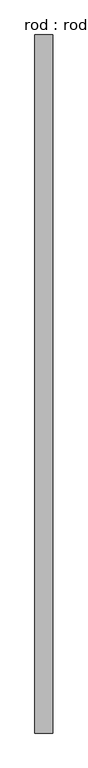
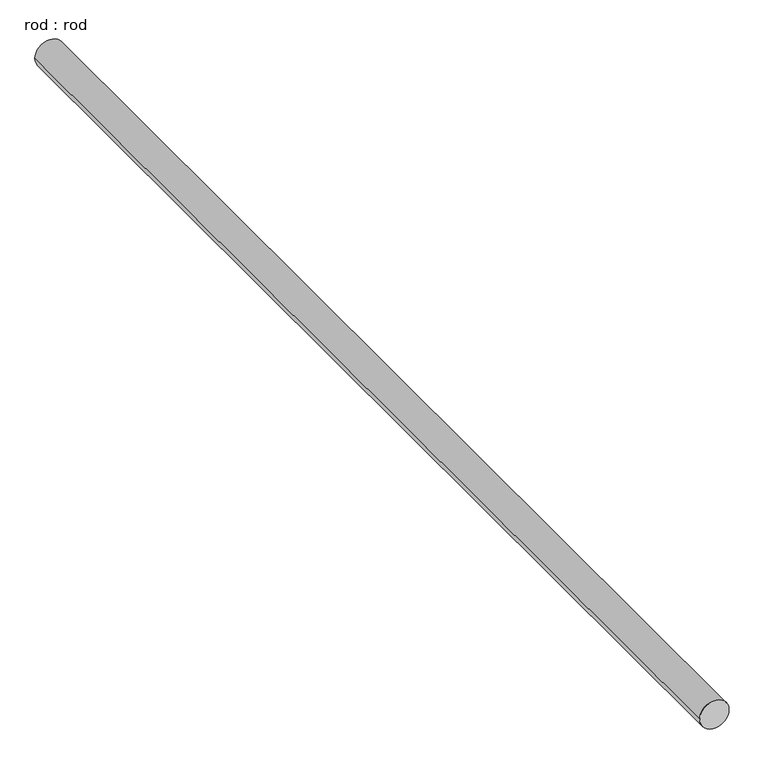
"""IFC4 building model written with IfcOpenShell, lengths in millimetres: proxy geometry, rod : rod."""

from ifc_helpers import new_model, si_unit, point, frame, frame_2d, origin, place, context, project, spatial, circle_curve, trimmed, segment, composite_curve, outline, extrude, source, transform, mapped, element, save


def rod_rod_e4fb1dad(model_context):
    return source(origin(), model_context, "Body", "SweptSolid", [
        extrude(outline(composite_curve([segment(trimmed(circle_curve(frame_2d((0.0108462, 0.0)), 200.0), [point((0.0108462, 200.0))], [point((0.0108462, -200.0))], False, "CARTESIAN"), True, "CONTINUOUS"), segment(trimmed(circle_curve(frame_2d((0.0108462, 0.0)), 200.0), [point((0.0108462, -200.0))], [point((0.0108462, 200.0))], False, "CARTESIAN"), True, "CONTINUOUS")], self_intersect=False)), frame((0.0, -3795.6642418, 0.0), z_axis=(0.0, 1.0, 0.0), x_axis=(0.0, 0.0, 1.0)), (0.0, 0.0, 1.0), 15776.7857143),
    ])


if __name__ == "__main__":
    model = new_model("IFC4")
    model_context = context("Model", 3, world=origin())
    ifc_project = project(units=[si_unit("LENGTHUNIT", "METRE", prefix="MILLI")], contexts=[model_context])
    site = spatial("IfcSite", under=ifc_project)
    building = spatial("IfcBuilding", under=site)
    placement = place(None, origin())
    rod_rod_shape = rod_rod_e4fb1dad(model_context)
    element("IfcBuildingElementProxy", 1, Name="rod : rod", ObjectType="rod : rod", at=placement, inside=building, context=model_context, shape_type="MappedRepresentation", body=[
        mapped(rod_rod_shape, transform((0.0, 0.0, 0.0), x_axis=(1.0, 0.0, 0.0), y_axis=(0.0, 1.0, 0.0), z_axis=(0.0, 0.0, 1.0))),
    ])
    save(model, "model.ifc")

# Revit data of these elements
# Type "rod : rod"
#   Default Elevation = 0
